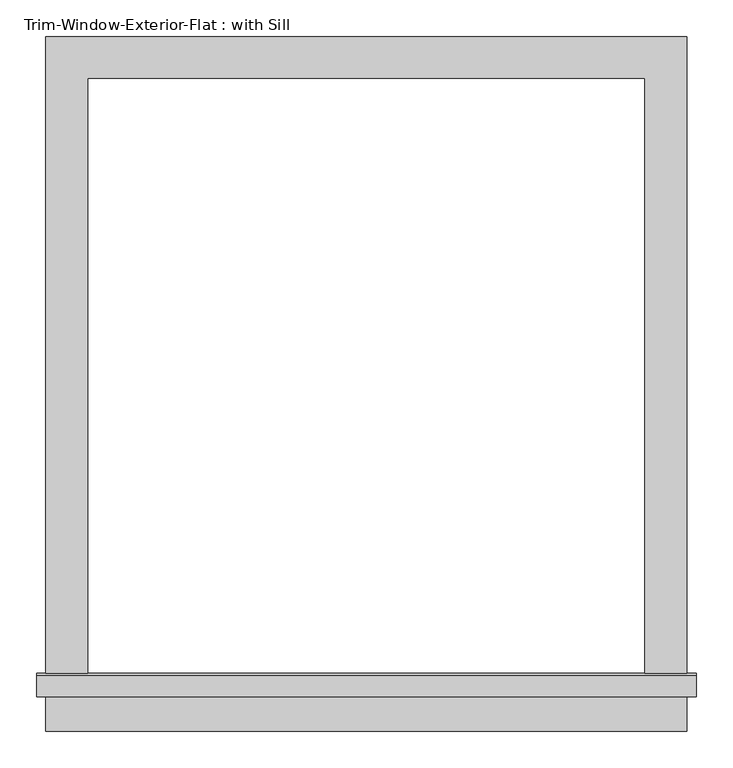
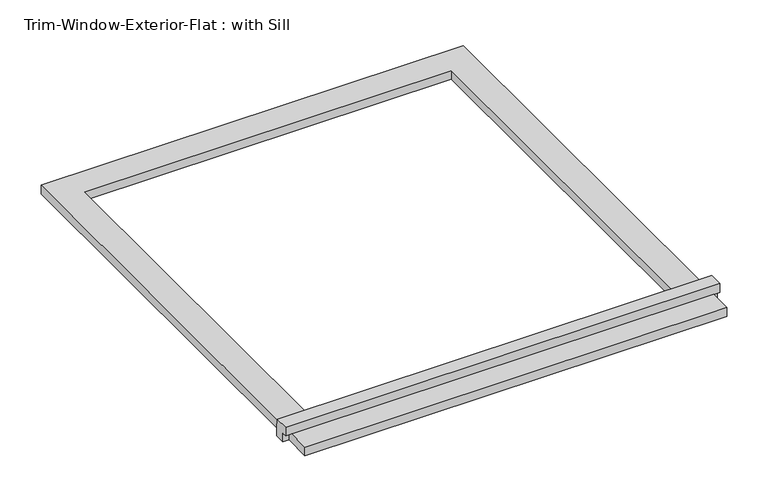
"""IFC4 building model written with IfcOpenShell, lengths in millimetres: proxy geometry, Trim-Window-Exterior-Flat : with Sill."""

from ifc_helpers import new_model, si_unit, frame, origin, origin_with_axes, place, context, project, spatial, polyline, outline, extrude, source, transform, mapped, element, save


def trim_window_exterior_flat_with_sill_9325c487(model_context):
    return source(origin(), model_context, "Body", "SweptSolid", [
        extrude(outline(polyline([(438.15, -834.9823709), (438.15, -892.1323709), (-438.15, -892.1323709), (-438.15, -834.9823709), (438.15, -834.9823709)])), origin_with_axes(), (0.0, 0.0, 1.0), 19.05),
        extrude(outline(polyline([(-844.55, 38.1), (-815.2580645, 38.1), (-812.8, 19.05), (-812.8, 0.0), (-834.9823709, 0.0), (-834.9823709, 19.05), (-844.55, 19.05), (-844.55, 38.1)])), frame((-450.85, 0.0, 0.0), z_axis=(1.0, 0.0, 0.0), x_axis=(0.0, 1.0, 0.0)), (0.0, 0.0, 1.0), 901.7),
        extrude(outline(polyline([(-438.15, 57.15), (438.15, 57.15), (438.15, -812.8), (381.0, -812.8), (381.0, 0.0), (-381.0, 0.0), (-381.0, -812.8), (-438.15, -812.8), (-438.15, 57.15)])), origin_with_axes(), (0.0, 0.0, 1.0), 19.05),
    ])


if __name__ == "__main__":
    model = new_model("IFC4")
    model_context = context("Model", 3, world=origin())
    ifc_project = project(units=[si_unit("LENGTHUNIT", "METRE", prefix="MILLI")], contexts=[model_context])
    site = spatial("IfcSite", under=ifc_project)
    building = spatial("IfcBuilding", under=site)
    placement = place(None, origin())
    trim_window_exterior_flat_with_sill_shape = trim_window_exterior_flat_with_sill_9325c487(model_context)
    element("IfcBuildingElementProxy", 1, Name="Trim-Window-Exterior-Flat : with Sill", ObjectType="Trim-Window-Exterior-Flat : with Sill", at=placement, inside=building, context=model_context, shape_type="MappedRepresentation", body=[
        mapped(trim_window_exterior_flat_with_sill_shape, transform((0.0, 0.0, 0.0), x_axis=(1.0, 0.0, 0.0), y_axis=(0.0, 1.0, 0.0), z_axis=(0.0, 0.0, 1.0))),
    ])
    save(model, "model.ifc")

# Revit data of these elements
# Type "Trim-Window-Exterior-Flat : with Sill"
#   Trim Width = 0' - 2 1/4"
#   Trim Thickness_Picture Frame = 0' - 1 1/4"
#   Trim Thickness_with Sill = 0' - 0 3/4"
#   Sill Thickness = 0' - 1 1/4"
#   Opening Width [instance default] = 2' - 0"
#   Opening Height [instance default] = 3' - 0"
#   Default Elevation = 4' - 0"
#   Sill = yes
#   Picture Frame = no
#   Trim Material [instance default] = none
# Element 1 (IfcBuildingElementProxy, "Trim-Window-Exterior-Flat : with Sill")
#   Opening Width = 2' - 6"
#   Opening Height = 2' - 8"
#   Trim Material = Clad - White
#   Materials on its faces: "Clad - White"
# Materials
#   "Clad - White": class "Wood", colour RGB 242 242 238, transparency 0, Cost = 0
